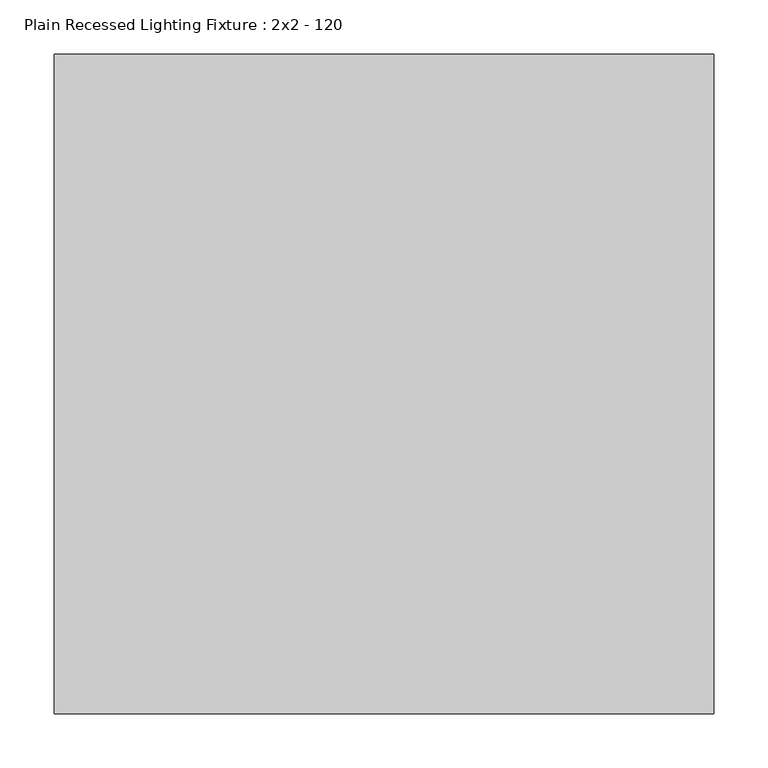
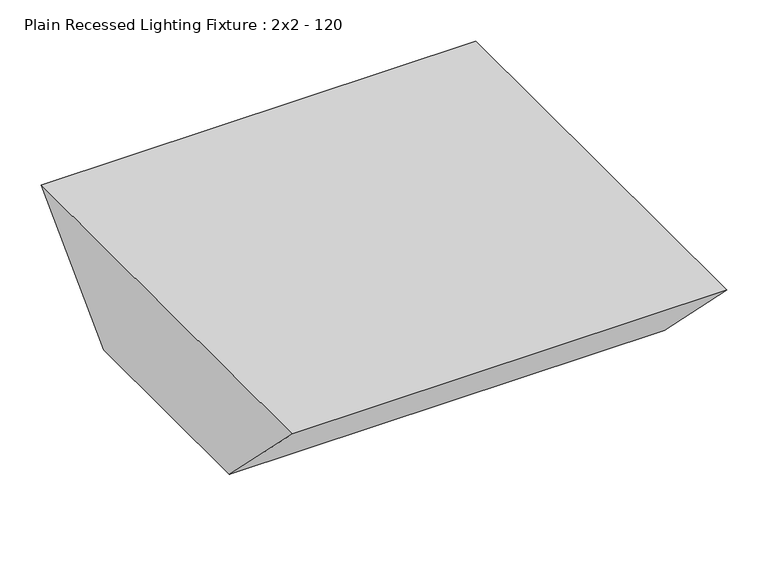
"""IFC4 building model written with IfcOpenShell, lengths in millimetres: light fixture geometry, Plain Recessed Lighting Fixture : 2x2 - 120."""

from ifc_helpers import new_model, si_unit, frame, origin, place, context, project, spatial, polyline, outline, extrude, source, transform, mapped, element, save


def plain_recessed_lighting_fixture_2x2_120_2107ce2d(model_context):
    return source(origin(), model_context, "Body", "SweptSolid", [
        extrude(outline(polyline([(-609.6, 0.0), (0.0, 0.0), (-152.4, -152.4), (-457.2, -152.4), (-609.6, 0.0)])), frame((0.0, 0.0, 0.0), z_axis=(1.0, 0.0, 0.0), x_axis=(0.0, 1.0, 0.0)), (0.0, 0.0, 1.0), 609.6),
    ])


if __name__ == "__main__":
    model = new_model("IFC4")
    model_context = context("Model", 3, world=origin())
    ifc_project = project(units=[si_unit("LENGTHUNIT", "METRE", prefix="MILLI")], contexts=[model_context])
    site = spatial("IfcSite", under=ifc_project)
    building = spatial("IfcBuilding", under=site)
    placement = place(None, origin())
    plain_recessed_lighting_fixture_2x2_120_shape = plain_recessed_lighting_fixture_2x2_120_2107ce2d(model_context)
    element("IfcLightFixture", 1, ObjectType="Plain Recessed Lighting Fixture : 2x2 - 120", at=placement, inside=building, context=model_context, shape_type="MappedRepresentation", body=[
        mapped(plain_recessed_lighting_fixture_2x2_120_shape, transform((0.0, 0.0, 0.0), x_axis=(1.0, 0.0, 0.0), y_axis=(0.0, 1.0, 0.0), z_axis=(0.0, 0.0, 1.0))),
    ])
    save(model, "model.ifc")

# Revit data of these elements
# Type "Plain Recessed Lighting Fixture : 2x2 - 120"
#   Photometric Web File = "2x22UA12.ies"
#   Width = 2' - 0"
#   Wattage = 62 W
#   built-in parameter 1150110 = 1 (stored number, unit not read)
#   built-in parameter 1150109 = 1 (stored number, unit not read)
#   built-in parameter 1150113 = 1 (stored number, unit not read)
#   Tilt Angle = -90.00°
#   Lumens = 5199.94 lm
#   built-in parameter 1114217 = 0.88 (stored number, unit not read)
#   built-in parameter 1150115 = 1 (stored number, unit not read)
#   built-in parameter 1150105 = 413.798 (stored number, unit not read)
#   Length = 2' - 0"
#   built-in parameter 1150112 = 1 (stored number, unit not read)
#   built-in parameter 1150114 = 1 (stored number, unit not read)
#   built-in parameter 1150107 = 4230 (stored number, unit not read)
#   built-in parameter 1150106 = 4.13798 (stored number, unit not read)
#   Emit from Rectangle Width = 2' - 0"
#   Emit from Rectangle Length = 2' - 0"
#   built-in parameter 1150104 = 7.79178 (stored number, unit not read)
#   Depth = 0' - 6"
#   Default Elevation = 4' - 0"
#   Ballast Voltage = 120 V
#   built-in parameter 1114218 = 0.88 (stored number, unit not read)
#   built-in parameter 1150133 = 10 (stored number, unit not read)
#   Apparent Load = 62 VA
#   built-in parameter 1150134 = 8
#   built-in parameter 1150137 = 1
#   Color Filter = 16777215
#   built-in parameter 1140040 [instance default] = 1
#   Load Classification = Lighting - Dwelling Unit
#   Emit Shape Visible in Rendering = no
#   Dimming Lamp Color Temperature Shift = (empty or 0)
#   Assembly Code = ""
